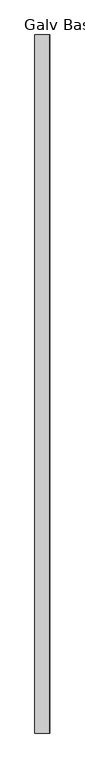
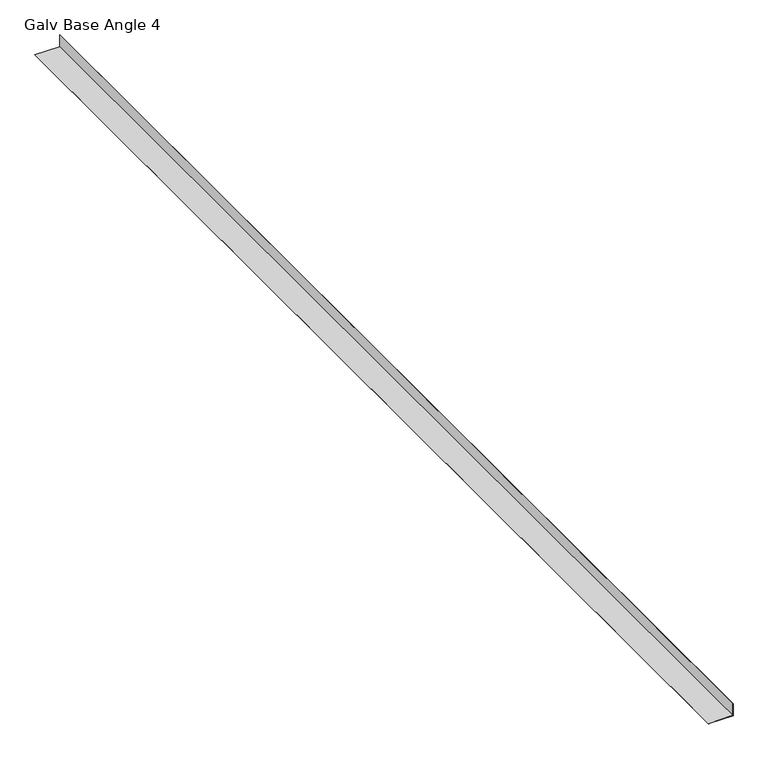
"""IFC4 building model written with IfcOpenShell, lengths in millimetres: proxy geometry, Galv Base Angle 4 : CF Galv L 4x2x16ga."""

from ifc_helpers import new_model, si_unit, frame, origin, place, context, project, spatial, polyline, outline, extrude, source, transform, mapped, element, save


def galv_base_angle_4_de8a329e(model_context):
    return source(origin(), model_context, "Body", "SweptSolid", [
        extrude(outline(polyline([(0.93726, 590250.3936739), (0.0, 590250.3936739), (0.0, 590351.9936739), (50.8, 590351.9936739), (50.8, 590351.0564139), (0.93726, 590351.0564139), (0.93726, 590250.3936739)])), frame((0.0, -536417.5913841, 0.0), z_axis=(0.0, 1.0, 0.0), x_axis=(0.0, 0.0, 1.0)), (0.0, 0.0, 1.0), 4743.45),
    ])


if __name__ == "__main__":
    model = new_model("IFC4")
    model_context = context("Model", 3, world=origin())
    ifc_project = project(units=[si_unit("LENGTHUNIT", "METRE", prefix="MILLI")], contexts=[model_context])
    site = spatial("IfcSite", under=ifc_project)
    building = spatial("IfcBuilding", under=site)
    placement = place(None, origin())
    galv_base_angle_4_shape = galv_base_angle_4_de8a329e(model_context)
    element("IfcBuildingElementProxy", 1, Name="Galv Base Angle 4 : CF Galv L 4x2x16ga", ObjectType="Galv Base Angle 4 : CF Galv L 4x2x16ga", at=placement, inside=building, context=model_context, shape_type="MappedRepresentation", body=[
        mapped(galv_base_angle_4_shape, transform((0.0, 0.0, 0.0), x_axis=(1.0, 0.0, 0.0), y_axis=(0.0, 1.0, 0.0), z_axis=(0.0, 0.0, 1.0))),
    ])
    save(model, "model.ifc")

# Revit data of these elements
# Element 1 (IfcBuildingElementProxy, "Galv Base Angle 4 : CF Galv L 4x2x16ga")
#   Materials on its faces: "4\"X2\" L - COLD-FORMED GALV."
# Materials
#   "4\"X2\" L - COLD-FORMED GALV.": class "Generic", colour RGB 143 142 141, transparency 0, Cost = 0
